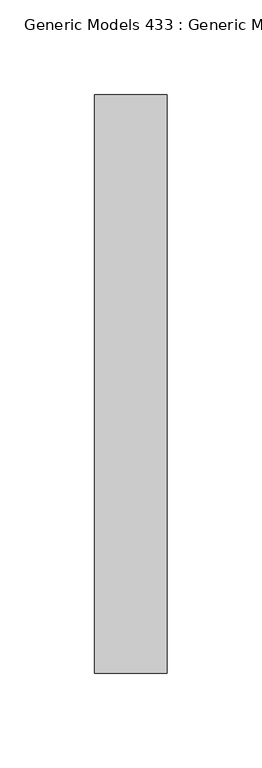
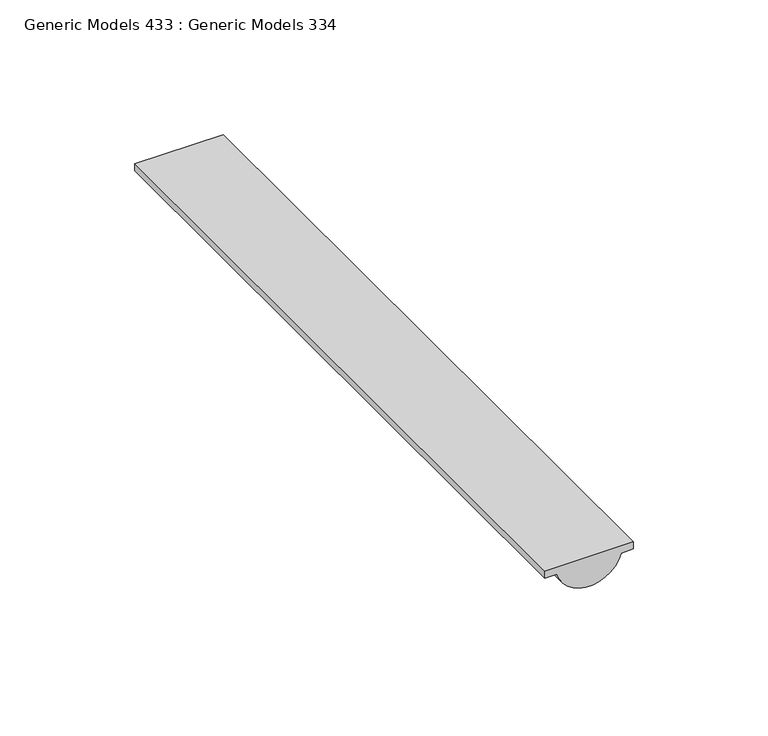
"""IFC4 building model written with IfcOpenShell, lengths in millimetres: proxy geometry, Generic Models 433 : Generic Models 334."""

import ifcopenshell
import ifcopenshell.guid

model = None  # the IFC model being written
_history = None  # IfcOwnerHistory: only IFC2X3 demands one
_inside = {}  # id of a spatial element -> (the spatial element, [elements in it])
_under = {}  # id of a project, library or spatial element -> (it, [spatial elements below it])
_declared = {}  # id of a project -> (the project, [libraries it declares])
_typed = {}  # id of a type object -> (the type object, [elements of that type])
_made_of = {}  # id of a material, layer set ... -> (it, [elements and type objects made of it])


def new_model(schema):
    """Start an empty IFC model of exactly this schema.

    Asked for "IFC4X3", IfcOpenShell would pick the latest addendum, in which some entities
    have other attributes; the version numbers below select the first issue.
    IFC2X3 requires an IfcOwnerHistory on every rooted entity: one is made here for all.
    """
    global model, _history
    if schema == "IFC4X3":
        model = ifcopenshell.file(schema_version=(4, 3, 0, 0))
    else:
        model = ifcopenshell.file(schema=schema)
    _inside.clear()
    _under.clear()
    _declared.clear()
    _typed.clear()
    _made_of.clear()
    _history = None
    if model.schema == "IFC2X3":
        org = make("IfcOrganization", Name="unknown")
        user = make(
            "IfcPersonAndOrganization",
            ThePerson=make("IfcPerson", FamilyName="unknown"),
            TheOrganization=org,
        )
        app = make(
            "IfcApplication",
            ApplicationDeveloper=org,
            Version="unknown",
            ApplicationFullName="unknown",
            ApplicationIdentifier="unknown",
        )
        _history = make(
            "IfcOwnerHistory",
            OwningUser=user,
            OwningApplication=app,
            ChangeAction="ADDED",
            CreationDate=0,
        )
    return model


def make(cls, **values):
    """One entity of the class cls with the attributes given. An attribute that is None is left unset."""
    return model.create_entity(
        cls, **{name: value for name, value in values.items() if value is not None}
    )


def rooted(cls, **values):
    """An entity with a GlobalId (a new one), such as an element, a storey or a relation."""
    return make(cls, GlobalId=ifcopenshell.guid.new(), OwnerHistory=_history, **values)


def si_unit(unit_type, name, prefix=None):
    """IfcSIUnit, for example si_unit("LENGTHUNIT", "METRE", prefix="MILLI")."""
    return make("IfcSIUnit", UnitType=unit_type, Prefix=prefix, Name=name)


def assignment(units):
    """IfcUnitAssignment: the units of a project."""
    return None if units is None else make("IfcUnitAssignment", Units=units)


def point(xyz):
    """IfcCartesianPoint."""
    return None if xyz is None else make("IfcCartesianPoint", Coordinates=xyz)


def direction(xyz):
    """IfcDirection."""
    return None if xyz is None else make("IfcDirection", DirectionRatios=xyz)


def frame(location, z_axis=None, x_axis=None):
    """IfcAxis2Placement3D, a coordinate frame: its origin and axes. An axis left out is left unset."""
    return make(
        "IfcAxis2Placement3D",
        Location=point(location),
        Axis=direction(z_axis),
        RefDirection=direction(x_axis),
    )


def frame_2d(location, x_axis=None):
    """IfcAxis2Placement2D, a coordinate frame in the plane: its origin and x axis."""
    return make(
        "IfcAxis2Placement2D", Location=point(location), RefDirection=direction(x_axis)
    )


def origin():
    """The frame at (0, 0, 0) with its axes left unset."""
    return frame((0.0, 0.0, 0.0))


def place(relative_to, where):
    """IfcLocalPlacement: puts the frame where relative to a parent placement (None: the world)."""
    return make(
        "IfcLocalPlacement", PlacementRelTo=relative_to, RelativePlacement=where
    )


def context(
    kind, dimensions, precision=None, world=None, true_north=None, identifier=None
):
    """IfcGeometricRepresentationContext, for example the 3D "Model" context."""
    return make(
        "IfcGeometricRepresentationContext",
        ContextIdentifier=identifier,
        ContextType=kind,
        CoordinateSpaceDimension=dimensions,
        Precision=precision,
        WorldCoordinateSystem=world,
        TrueNorth=true_north,
    )


def project(units=None, contexts=None):
    """IfcProject with its units and contexts."""
    return rooted(
        "IfcProject",
        Name="project",
        RepresentationContexts=contexts,
        UnitsInContext=assignment(units),
    )


def spatial(cls, under=None, at=None, **own):
    """A site, building, storey or space (cls), placed at a placement, below another one or the project."""
    s = rooted(cls, ObjectPlacement=at, **own)
    if under is not None:
        _under.setdefault(under.id(), (under, []))[1].append(s)
    return s


def polyline(points):
    """IfcPolyline through the points."""
    return make("IfcPolyline", Points=[point(p) for p in points])


def circle_curve(where, radius):
    """IfcCircle in the frame where."""
    return make("IfcCircle", Position=where, Radius=radius)


def trimmed(basis, trim1, trim2, sense, master):
    """IfcTrimmedCurve: the piece of a basis curve between two trims."""
    return make(
        "IfcTrimmedCurve",
        BasisCurve=basis,
        Trim1=trim1,
        Trim2=trim2,
        SenseAgreement=sense,
        MasterRepresentation=master,
    )


def segment(curve, same_sense, transition):
    """IfcCompositeCurveSegment."""
    return make(
        "IfcCompositeCurveSegment",
        Transition=transition,
        SameSense=same_sense,
        ParentCurve=curve,
    )


def composite_curve(segments, self_intersect=None):
    """IfcCompositeCurve: segments joined end to end."""
    return make("IfcCompositeCurve", Segments=segments, SelfIntersect=self_intersect)


def outline(outer, holes=None, kind="AREA"):
    """IfcArbitraryClosedProfileDef: a profile drawn as a closed curve; with holes, ...WithVoids."""
    if holes is None:
        return make("IfcArbitraryClosedProfileDef", ProfileType=kind, OuterCurve=outer)
    return make(
        "IfcArbitraryProfileDefWithVoids",
        ProfileType=kind,
        OuterCurve=outer,
        InnerCurves=holes,
    )


def extrude(swept, where, along, depth):
    """IfcExtrudedAreaSolid: the profile swept, set in the frame where, extruded along a direction by depth."""
    return make(
        "IfcExtrudedAreaSolid",
        SweptArea=swept,
        Position=where,
        ExtrudedDirection=direction(along),
        Depth=depth,
    )


def shape(context_of_items, identifier, shape_type, items):
    """IfcShapeRepresentation: the items that make up one representation, for example the "Body"."""
    return make(
        "IfcShapeRepresentation",
        ContextOfItems=context_of_items,
        RepresentationIdentifier=identifier,
        RepresentationType=shape_type,
        Items=items,
    )


def source(mapping_origin, context_of_items, identifier, shape_type, items):
    """IfcRepresentationMap: a shape defined once, which mapped items show again and again."""
    return make(
        "IfcRepresentationMap",
        MappingOrigin=mapping_origin,
        MappedRepresentation=shape(context_of_items, identifier, shape_type, items),
    )


def transform(
    local_origin,
    x_axis=None,
    y_axis=None,
    z_axis=None,
    scale=None,
    scale2=None,
    scale3=None,
    uniform=True,
):
    """IfcCartesianTransformationOperator3D, or its non-uniform kind. x_axis, y_axis, z_axis: its Axis1, 2, 3."""
    if uniform:
        return make(
            "IfcCartesianTransformationOperator3D",
            Axis1=direction(x_axis),
            Axis2=direction(y_axis),
            LocalOrigin=point(local_origin),
            Scale=scale,
            Axis3=direction(z_axis),
        )
    return make(
        "IfcCartesianTransformationOperator3DnonUniform",
        Axis1=direction(x_axis),
        Axis2=direction(y_axis),
        LocalOrigin=point(local_origin),
        Scale=scale,
        Axis3=direction(z_axis),
        Scale2=scale2,
        Scale3=scale3,
    )


def mapped(mapping_source, mapping_target):
    """IfcMappedItem: shows the shape of a source again, moved by a transform."""
    return make(
        "IfcMappedItem", MappingSource=mapping_source, MappingTarget=mapping_target
    )


def made_of(thing, what):
    """Note that an element or type object is made of a material, layer set ...; save() writes the relation."""
    if what is not None:
        _made_of.setdefault(what.id(), (what, []))[1].append(thing)
    return thing


def element(
    cls,
    number,
    at=None,
    inside=None,
    cuts=None,
    type_object=None,
    material=None,
    context=None,
    identifier="Body",
    shape_type=None,
    held_by="IfcProductDefinitionShape",
    body=None,
    shapes=None,
    **own,
):
    """One element of the class cls, such as IfcWall. Its Tag is "e" and its number.

    at: its placement. inside: the storey or other place that contains it. cuts: it is an
    opening in that element (IfcRelVoidsElement). A single representation is given by context,
    identifier, shape_type and body (its items); several are given by shapes. held_by: the class
    of the entity that holds the representations. save() writes the other relations.
    """
    e = rooted(cls, Tag="e%d" % number, ObjectPlacement=at, **own)
    if body is not None:
        shapes = [shape(context, identifier, shape_type, body)]
    if shapes is not None:
        e.Representation = make(held_by, Representations=shapes)
    if inside is not None:
        _inside.setdefault(inside.id(), (inside, []))[1].append(e)
    if cuts is not None:
        rooted(
            "IfcRelVoidsElement", RelatingBuildingElement=cuts, RelatedOpeningElement=e
        )
    if type_object is not None:
        _typed.setdefault(type_object.id(), (type_object, []))[1].append(e)
    return made_of(e, material)


def aggregate(whole, parts):
    """IfcRelAggregates: a whole, such as a stair, and the parts it consists of."""
    return rooted("IfcRelAggregates", RelatingObject=whole, RelatedObjects=parts)


def save(model, path):
    """Write the relations noted so far, then the file.

    IfcRelAggregates (storeys below a building ...), IfcRelContainedInSpatialStructure (elements
    in a storey), IfcRelDefinesByType, IfcRelAssociatesMaterial and IfcRelDeclares: one each for
    every whole, place, type object, material and project.
    """
    for whole, parts in _under.values():
        aggregate(whole, parts)
    for where, things in _inside.values():
        rooted(
            "IfcRelContainedInSpatialStructure",
            RelatedElements=things,
            RelatingStructure=where,
        )
    for kind, things in _typed.values():
        rooted("IfcRelDefinesByType", RelatedObjects=things, RelatingType=kind)
    for what, things in _made_of.values():
        rooted("IfcRelAssociatesMaterial", RelatedObjects=things, RelatingMaterial=what)
    for by, libraries in _declared.values():
        rooted("IfcRelDeclares", RelatingContext=by, RelatedDefinitions=libraries)
    model.write(path)


def generic_models_433_generic_models_334_03cef7c8(model_context):
    return source(origin(), model_context, "Body", "SweptSolid", [
        extrude(outline(composite_curve([segment(polyline([(123781.5216496, 8247.7371996), (123778.3466496, 8247.7371996), (123778.3466496, 8252.951842)]), True, "CONTINUOUS"), segment(trimmed(circle_curve(frame_2d((123782.4661193, 8266.7871996)), 14.4356208), [point((123778.3466496, 8252.951842))], [point((123778.3466496, 8280.6225572))], False, "CARTESIAN"), True, "CONTINUOUS"), segment(polyline([(123778.3466496, 8280.6225572), (123778.3466496, 8285.8371996), (123781.5216496, 8285.8371996), (123781.5216496, 8247.7371996)]), True, "CONTINUOUS")], self_intersect=False)), frame((0.0, -4109.6428838, 0.0), z_axis=(0.0, 1.0, 0.0), x_axis=(0.0, 0.0, 1.0)), (0.0, 0.0, 1.0), 304.8),
    ])


if __name__ == "__main__":
    model = new_model("IFC4")
    model_context = context("Model", 3, world=origin())
    ifc_project = project(units=[si_unit("LENGTHUNIT", "METRE", prefix="MILLI")], contexts=[model_context])
    site = spatial("IfcSite", under=ifc_project)
    building = spatial("IfcBuilding", under=site)
    placement = place(None, origin())
    generic_models_433_generic_models_334_shape = generic_models_433_generic_models_334_03cef7c8(model_context)
    element("IfcBuildingElementProxy", 1, Name="Generic Models 433 : Generic Models 334", ObjectType="Generic Models 433 : Generic Models 334", at=placement, inside=building, context=model_context, shape_type="MappedRepresentation", body=[
        mapped(generic_models_433_generic_models_334_shape, transform((0.0, 0.0, 0.0), x_axis=(1.0, 0.0, 0.0), y_axis=(0.0, 1.0, 0.0), z_axis=(0.0, 0.0, 1.0))),
    ])
    save(model, "model.ifc")

# Revit data of these elements
# Element 1 (IfcBuildingElementProxy, "Generic Models 433 : Generic Models 334")
#   Materials on its faces: "_WEATHER STRIPPING"
# Materials
#   "_WEATHER STRIPPING": class "Generic", colour RGB 245 226 173, transparency 0, Cost = 0
